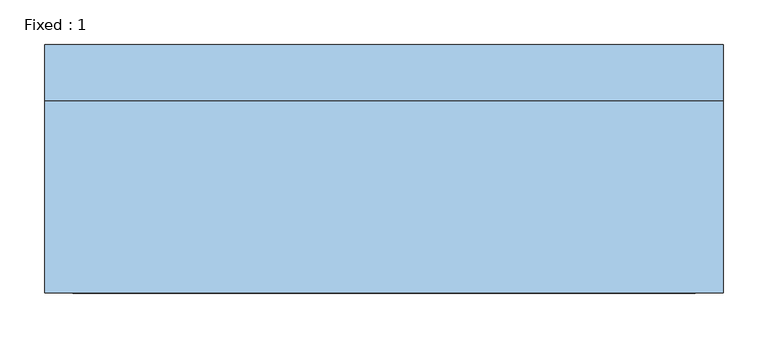
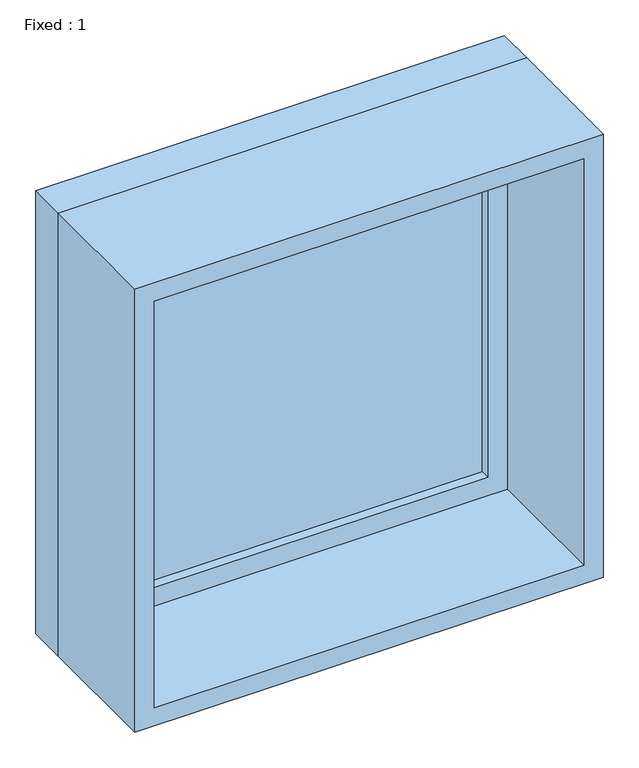
"""IFC4 building model written with IfcOpenShell, lengths in millimetres: window geometry, Fixed : 1."""

import ifcopenshell
import ifcopenshell.guid

model = None  # the IFC model being written
_history = None  # IfcOwnerHistory: only IFC2X3 demands one
_inside = {}  # id of a spatial element -> (the spatial element, [elements in it])
_under = {}  # id of a project, library or spatial element -> (it, [spatial elements below it])
_declared = {}  # id of a project -> (the project, [libraries it declares])
_typed = {}  # id of a type object -> (the type object, [elements of that type])
_made_of = {}  # id of a material, layer set ... -> (it, [elements and type objects made of it])


def new_model(schema):
    """Start an empty IFC model of exactly this schema.

    Asked for "IFC4X3", IfcOpenShell would pick the latest addendum, in which some entities
    have other attributes; the version numbers below select the first issue.
    IFC2X3 requires an IfcOwnerHistory on every rooted entity: one is made here for all.
    """
    global model, _history
    if schema == "IFC4X3":
        model = ifcopenshell.file(schema_version=(4, 3, 0, 0))
    else:
        model = ifcopenshell.file(schema=schema)
    _inside.clear()
    _under.clear()
    _declared.clear()
    _typed.clear()
    _made_of.clear()
    _history = None
    if model.schema == "IFC2X3":
        org = make("IfcOrganization", Name="unknown")
        user = make(
            "IfcPersonAndOrganization",
            ThePerson=make("IfcPerson", FamilyName="unknown"),
            TheOrganization=org,
        )
        app = make(
            "IfcApplication",
            ApplicationDeveloper=org,
            Version="unknown",
            ApplicationFullName="unknown",
            ApplicationIdentifier="unknown",
        )
        _history = make(
            "IfcOwnerHistory",
            OwningUser=user,
            OwningApplication=app,
            ChangeAction="ADDED",
            CreationDate=0,
        )
    return model


def make(cls, **values):
    """One entity of the class cls with the attributes given. An attribute that is None is left unset."""
    return model.create_entity(
        cls, **{name: value for name, value in values.items() if value is not None}
    )


def rooted(cls, **values):
    """An entity with a GlobalId (a new one), such as an element, a storey or a relation."""
    return make(cls, GlobalId=ifcopenshell.guid.new(), OwnerHistory=_history, **values)


def si_unit(unit_type, name, prefix=None):
    """IfcSIUnit, for example si_unit("LENGTHUNIT", "METRE", prefix="MILLI")."""
    return make("IfcSIUnit", UnitType=unit_type, Prefix=prefix, Name=name)


def assignment(units):
    """IfcUnitAssignment: the units of a project."""
    return None if units is None else make("IfcUnitAssignment", Units=units)


def point(xyz):
    """IfcCartesianPoint."""
    return None if xyz is None else make("IfcCartesianPoint", Coordinates=xyz)


def direction(xyz):
    """IfcDirection."""
    return None if xyz is None else make("IfcDirection", DirectionRatios=xyz)


def frame(location, z_axis=None, x_axis=None):
    """IfcAxis2Placement3D, a coordinate frame: its origin and axes. An axis left out is left unset."""
    return make(
        "IfcAxis2Placement3D",
        Location=point(location),
        Axis=direction(z_axis),
        RefDirection=direction(x_axis),
    )


def origin():
    """The frame at (0, 0, 0) with its axes left unset."""
    return frame((0.0, 0.0, 0.0))


def place(relative_to, where):
    """IfcLocalPlacement: puts the frame where relative to a parent placement (None: the world)."""
    return make(
        "IfcLocalPlacement", PlacementRelTo=relative_to, RelativePlacement=where
    )


def context(
    kind, dimensions, precision=None, world=None, true_north=None, identifier=None
):
    """IfcGeometricRepresentationContext, for example the 3D "Model" context."""
    return make(
        "IfcGeometricRepresentationContext",
        ContextIdentifier=identifier,
        ContextType=kind,
        CoordinateSpaceDimension=dimensions,
        Precision=precision,
        WorldCoordinateSystem=world,
        TrueNorth=true_north,
    )


def project(units=None, contexts=None):
    """IfcProject with its units and contexts."""
    return rooted(
        "IfcProject",
        Name="project",
        RepresentationContexts=contexts,
        UnitsInContext=assignment(units),
    )


def spatial(cls, under=None, at=None, **own):
    """A site, building, storey or space (cls), placed at a placement, below another one or the project."""
    s = rooted(cls, ObjectPlacement=at, **own)
    if under is not None:
        _under.setdefault(under.id(), (under, []))[1].append(s)
    return s


def polyline(points):
    """IfcPolyline through the points."""
    return make("IfcPolyline", Points=[point(p) for p in points])


def outline(outer, holes=None, kind="AREA"):
    """IfcArbitraryClosedProfileDef: a profile drawn as a closed curve; with holes, ...WithVoids."""
    if holes is None:
        return make("IfcArbitraryClosedProfileDef", ProfileType=kind, OuterCurve=outer)
    return make(
        "IfcArbitraryProfileDefWithVoids",
        ProfileType=kind,
        OuterCurve=outer,
        InnerCurves=holes,
    )


def extrude(swept, where, along, depth):
    """IfcExtrudedAreaSolid: the profile swept, set in the frame where, extruded along a direction by depth."""
    return make(
        "IfcExtrudedAreaSolid",
        SweptArea=swept,
        Position=where,
        ExtrudedDirection=direction(along),
        Depth=depth,
    )


def shape(context_of_items, identifier, shape_type, items):
    """IfcShapeRepresentation: the items that make up one representation, for example the "Body"."""
    return make(
        "IfcShapeRepresentation",
        ContextOfItems=context_of_items,
        RepresentationIdentifier=identifier,
        RepresentationType=shape_type,
        Items=items,
    )


def source(mapping_origin, context_of_items, identifier, shape_type, items):
    """IfcRepresentationMap: a shape defined once, which mapped items show again and again."""
    return make(
        "IfcRepresentationMap",
        MappingOrigin=mapping_origin,
        MappedRepresentation=shape(context_of_items, identifier, shape_type, items),
    )


def transform(
    local_origin,
    x_axis=None,
    y_axis=None,
    z_axis=None,
    scale=None,
    scale2=None,
    scale3=None,
    uniform=True,
):
    """IfcCartesianTransformationOperator3D, or its non-uniform kind. x_axis, y_axis, z_axis: its Axis1, 2, 3."""
    if uniform:
        return make(
            "IfcCartesianTransformationOperator3D",
            Axis1=direction(x_axis),
            Axis2=direction(y_axis),
            LocalOrigin=point(local_origin),
            Scale=scale,
            Axis3=direction(z_axis),
        )
    return make(
        "IfcCartesianTransformationOperator3DnonUniform",
        Axis1=direction(x_axis),
        Axis2=direction(y_axis),
        LocalOrigin=point(local_origin),
        Scale=scale,
        Axis3=direction(z_axis),
        Scale2=scale2,
        Scale3=scale3,
    )


def mapped(mapping_source, mapping_target):
    """IfcMappedItem: shows the shape of a source again, moved by a transform."""
    return make(
        "IfcMappedItem", MappingSource=mapping_source, MappingTarget=mapping_target
    )


def made_of(thing, what):
    """Note that an element or type object is made of a material, layer set ...; save() writes the relation."""
    if what is not None:
        _made_of.setdefault(what.id(), (what, []))[1].append(thing)
    return thing


def element(
    cls,
    number,
    at=None,
    inside=None,
    cuts=None,
    type_object=None,
    material=None,
    context=None,
    identifier="Body",
    shape_type=None,
    held_by="IfcProductDefinitionShape",
    body=None,
    shapes=None,
    **own,
):
    """One element of the class cls, such as IfcWall. Its Tag is "e" and its number.

    at: its placement. inside: the storey or other place that contains it. cuts: it is an
    opening in that element (IfcRelVoidsElement). A single representation is given by context,
    identifier, shape_type and body (its items); several are given by shapes. held_by: the class
    of the entity that holds the representations. save() writes the other relations.
    """
    e = rooted(cls, Tag="e%d" % number, ObjectPlacement=at, **own)
    if body is not None:
        shapes = [shape(context, identifier, shape_type, body)]
    if shapes is not None:
        e.Representation = make(held_by, Representations=shapes)
    if inside is not None:
        _inside.setdefault(inside.id(), (inside, []))[1].append(e)
    if cuts is not None:
        rooted(
            "IfcRelVoidsElement", RelatingBuildingElement=cuts, RelatedOpeningElement=e
        )
    if type_object is not None:
        _typed.setdefault(type_object.id(), (type_object, []))[1].append(e)
    return made_of(e, material)


def aggregate(whole, parts):
    """IfcRelAggregates: a whole, such as a stair, and the parts it consists of."""
    return rooted("IfcRelAggregates", RelatingObject=whole, RelatedObjects=parts)


def save(model, path):
    """Write the relations noted so far, then the file.

    IfcRelAggregates (storeys below a building ...), IfcRelContainedInSpatialStructure (elements
    in a storey), IfcRelDefinesByType, IfcRelAssociatesMaterial and IfcRelDeclares: one each for
    every whole, place, type object, material and project.
    """
    for whole, parts in _under.values():
        aggregate(whole, parts)
    for where, things in _inside.values():
        rooted(
            "IfcRelContainedInSpatialStructure",
            RelatedElements=things,
            RelatingStructure=where,
        )
    for kind, things in _typed.values():
        rooted("IfcRelDefinesByType", RelatedObjects=things, RelatingType=kind)
    for what, things in _made_of.values():
        rooted("IfcRelAssociatesMaterial", RelatedObjects=things, RelatingMaterial=what)
    for by, libraries in _declared.values():
        rooted("IfcRelDeclares", RelatingContext=by, RelatedDefinitions=libraries)
    model.write(path)


def fixed_1_cc56f13b(model_context):
    return source(origin(), model_context, "Body", "SweptSolid", [
        extrude(outline(polyline([(279.4, 92.075), (-355.6, 92.075), (-355.6, 104.775), (279.4, 104.775), (279.4, 92.075)])), frame((0.0, 0.0, 977.9), z_axis=(0.0, 0.0, 1.0), x_axis=(1.0, 0.0, 0.0)), (0.0, 0.0, 1.0), 635.0),
        extrude(outline(polyline([(1657.35, -400.05), (933.45, -400.05), (933.45, 323.85), (1657.35, 323.85), (1657.35, -400.05)]), holes=[polyline([(1612.9, -355.6), (1612.9, 279.4), (977.9, 279.4), (977.9, -355.6), (1612.9, -355.6)])]), frame((0.0, 76.2, 0.0), z_axis=(0.0, 1.0, 0.0), x_axis=(0.0, 0.0, 1.0)), (0.0, 0.0, 1.0), 44.45),
        extrude(outline(polyline([(1676.4, -419.1), (914.4, -419.1), (914.4, 342.9), (1676.4, 342.9), (1676.4, -419.1)]), holes=[polyline([(1644.65, -387.35), (1644.65, 311.15), (946.15, 311.15), (946.15, -387.35), (1644.65, -387.35)])]), frame((0.0, -139.7, 0.0), z_axis=(0.0, 1.0, 0.0), x_axis=(0.0, 0.0, 1.0)), (0.0, 0.0, 1.0), 215.9),
        extrude(outline(polyline([(1676.4, 342.9), (1676.4, -419.1), (914.4, -419.1), (914.4, 342.9), (1676.4, 342.9)]), holes=[polyline([(1657.35, 323.85), (933.45, 323.85), (933.45, -400.05), (1657.35, -400.05), (1657.35, 323.85)])]), frame((0.0, 76.2, 0.0), z_axis=(0.0, 1.0, 0.0), x_axis=(0.0, 0.0, 1.0)), (0.0, 0.0, 1.0), 63.5),
    ])


if __name__ == "__main__":
    model = new_model("IFC4")
    model_context = context("Model", 3, world=origin())
    ifc_project = project(units=[si_unit("LENGTHUNIT", "METRE", prefix="MILLI")], contexts=[model_context])
    site = spatial("IfcSite", under=ifc_project)
    building = spatial("IfcBuilding", under=site)
    placement = place(None, origin())
    fixed_1_shape = fixed_1_cc56f13b(model_context)
    element("IfcWindow", 1, ObjectType="Fixed : 1", at=placement, inside=building, context=model_context, shape_type="MappedRepresentation", body=[
        mapped(fixed_1_shape, transform((0.0, 0.0, 0.0), x_axis=(1.0, 0.0, 0.0), y_axis=(0.0, 1.0, 0.0), z_axis=(0.0, 0.0, 1.0))),
    ])
    save(model, "model.ifc")

# Revit data of these elements
# Type "Fixed : 1"
#   Type Mark = "11"
#   Assembly Code = "B2020100"
#   Height = 2' - 6"
#   Default Sill Height = 3' - 0"
#   Width = 2' - 6"
#   Window Inset = 0' - 0 3/4"
#   Glass Pane Material = Glass
#   Sash Material = accent 1
#   Wall Closure = (empty or 0)
# Element 1 (IfcWindow, "Fixed : 1")
#   Materials on its faces: "accent 1", "Glass"
# Materials
#   "Glass": class "Glass", colour RGB 236 240 239, transparency 0.85, Description = "Soda Lime Glass", Cost = 0
#   "accent 1": class "Generic", colour RGB 92 104 51, transparency 0, Cost = 0
